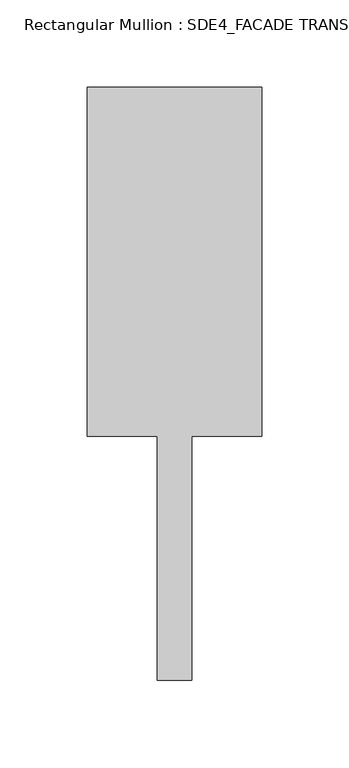
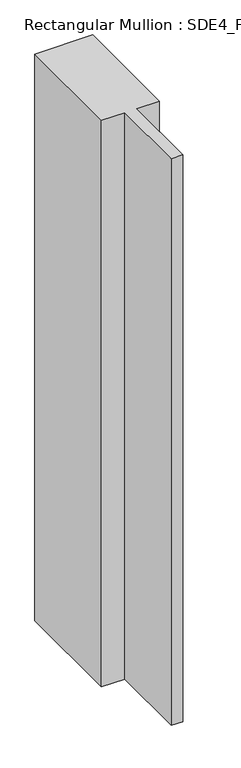
"""IFC4 building model written with IfcOpenShell, lengths in millimetres: member geometry, Rectangular Mullion : SDE4_FACADE TRANSOM TYPE 1."""

from ifc_helpers import new_model, si_unit, frame, origin, place, context, project, spatial, polyline, outline, extrude, source, transform, mapped, element, save


def rectangular_mullion_sde4_facade_transom_type_1_eb20d0a4(model_context):
    return source(origin(), model_context, "Body", "SweptSolid", [
        extrude(outline(polyline([(50.0, 132.5), (50.0, -67.5), (10.0, -67.5), (10.0, -207.5), (-10.0, -207.5), (-10.0, -67.5), (-50.0, -67.5), (-50.0, 132.5), (50.0, 132.5)])), frame((0.0, 0.0, -1039.0), z_axis=(0.0, 0.0, 1.0), x_axis=(1.0, 0.0, 0.0)), (0.0, 0.0, 1.0), 1039.0),
    ])


if __name__ == "__main__":
    model = new_model("IFC4")
    model_context = context("Model", 3, world=origin())
    ifc_project = project(units=[si_unit("LENGTHUNIT", "METRE", prefix="MILLI")], contexts=[model_context])
    site = spatial("IfcSite", under=ifc_project)
    building = spatial("IfcBuilding", under=site)
    placement = place(None, origin())
    rectangular_mullion_sde4_facade_transom_type_1_shape = rectangular_mullion_sde4_facade_transom_type_1_eb20d0a4(model_context)
    element("IfcMember", 1, ObjectType="Rectangular Mullion : SDE4_FACADE TRANSOM TYPE 1", at=placement, inside=building, context=model_context, shape_type="MappedRepresentation", body=[
        mapped(rectangular_mullion_sde4_facade_transom_type_1_shape, transform((0.0, 0.0, 0.0), x_axis=(1.0, 0.0, 0.0), y_axis=(0.0, 1.0, 0.0), z_axis=(0.0, 0.0, 1.0))),
    ])
    save(model, "model.ifc")

# Revit data of these elements
# Type "Rectangular Mullion : SDE4_FACADE TRANSOM TYPE 1"
#   built-in parameter 1007322 = 1.11549 (stored number, unit not read)
#   built-in parameter 1007321 = 0.164042 (stored number, unit not read)
#   built-in parameter 1007320 = 0.164042 (stored number, unit not read)
